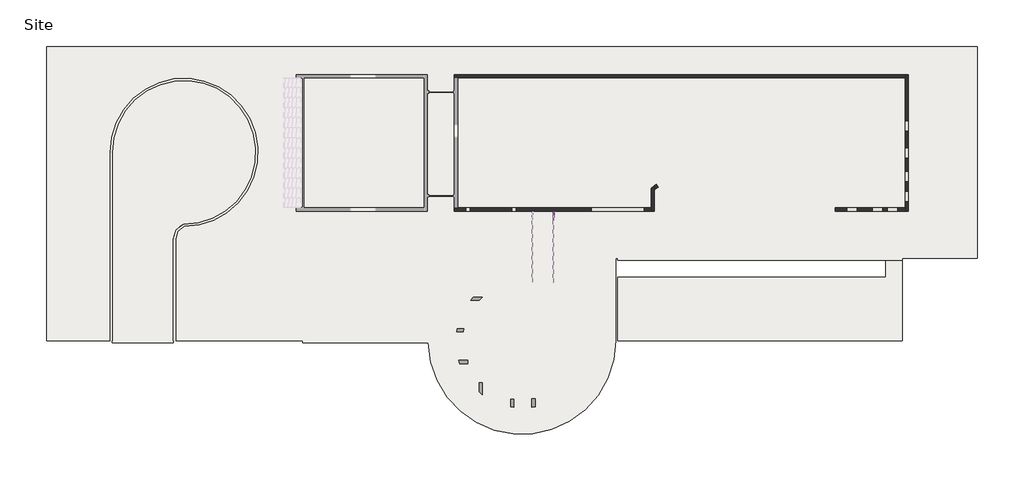
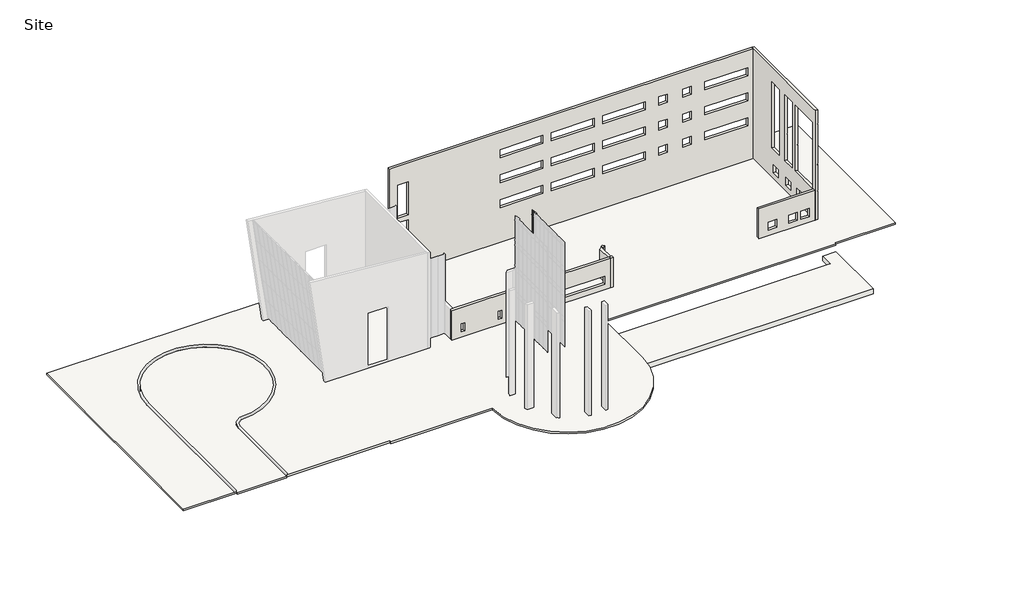
# One storey, part 4 of 4: 17 members, 6 walls, 3 plates, 3 slabs.
"""IFC4 building model written with IfcOpenShell, lengths in millimetres."""

import ifcopenshell
import ifcopenshell.guid

model = None  # the IFC model being written
_history = None  # IfcOwnerHistory: only IFC2X3 demands one
_inside = {}  # id of a spatial element -> (the spatial element, [elements in it])
_under = {}  # id of a project, library or spatial element -> (it, [spatial elements below it])
_declared = {}  # id of a project -> (the project, [libraries it declares])
_typed = {}  # id of a type object -> (the type object, [elements of that type])
_made_of = {}  # id of a material, layer set ... -> (it, [elements and type objects made of it])


def new_model(schema):
    """Start an empty IFC model of exactly this schema.

    Asked for "IFC4X3", IfcOpenShell would pick the latest addendum, in which some entities
    have other attributes; the version numbers below select the first issue.
    IFC2X3 requires an IfcOwnerHistory on every rooted entity: one is made here for all.
    """
    global model, _history
    if schema == "IFC4X3":
        model = ifcopenshell.file(schema_version=(4, 3, 0, 0))
    else:
        model = ifcopenshell.file(schema=schema)
    _inside.clear()
    _under.clear()
    _declared.clear()
    _typed.clear()
    _made_of.clear()
    _history = None
    if model.schema == "IFC2X3":
        org = make("IfcOrganization", Name="unknown")
        user = make(
            "IfcPersonAndOrganization",
            ThePerson=make("IfcPerson", FamilyName="unknown"),
            TheOrganization=org,
        )
        app = make(
            "IfcApplication",
            ApplicationDeveloper=org,
            Version="unknown",
            ApplicationFullName="unknown",
            ApplicationIdentifier="unknown",
        )
        _history = make(
            "IfcOwnerHistory",
            OwningUser=user,
            OwningApplication=app,
            ChangeAction="ADDED",
            CreationDate=0,
        )
    return model


def make(cls, **values):
    """One entity of the class cls with the attributes given. An attribute that is None is left unset."""
    return model.create_entity(
        cls, **{name: value for name, value in values.items() if value is not None}
    )


def rooted(cls, **values):
    """An entity with a GlobalId (a new one), such as an element, a storey or a relation."""
    return make(cls, GlobalId=ifcopenshell.guid.new(), OwnerHistory=_history, **values)


def si_unit(unit_type, name, prefix=None):
    """IfcSIUnit, for example si_unit("LENGTHUNIT", "METRE", prefix="MILLI")."""
    return make("IfcSIUnit", UnitType=unit_type, Prefix=prefix, Name=name)


def assignment(units):
    """IfcUnitAssignment: the units of a project."""
    return None if units is None else make("IfcUnitAssignment", Units=units)


def point(xyz):
    """IfcCartesianPoint."""
    return None if xyz is None else make("IfcCartesianPoint", Coordinates=xyz)


def direction(xyz):
    """IfcDirection."""
    return None if xyz is None else make("IfcDirection", DirectionRatios=xyz)


def frame(location, z_axis=None, x_axis=None):
    """IfcAxis2Placement3D, a coordinate frame: its origin and axes. An axis left out is left unset."""
    return make(
        "IfcAxis2Placement3D",
        Location=point(location),
        Axis=direction(z_axis),
        RefDirection=direction(x_axis),
    )


def frame_2d(location, x_axis=None):
    """IfcAxis2Placement2D, a coordinate frame in the plane: its origin and x axis."""
    return make(
        "IfcAxis2Placement2D", Location=point(location), RefDirection=direction(x_axis)
    )


def origin():
    """The frame at (0, 0, 0) with its axes left unset."""
    return frame((0.0, 0.0, 0.0))


def origin_with_axes():
    """The frame at (0, 0, 0) with the z axis (0, 0, 1) and the x axis (1, 0, 0) written out."""
    return frame((0.0, 0.0, 0.0), z_axis=(0.0, 0.0, 1.0), x_axis=(1.0, 0.0, 0.0))


def place(relative_to, where):
    """IfcLocalPlacement: puts the frame where relative to a parent placement (None: the world)."""
    return make(
        "IfcLocalPlacement", PlacementRelTo=relative_to, RelativePlacement=where
    )


def context(
    kind, dimensions, precision=None, world=None, true_north=None, identifier=None
):
    """IfcGeometricRepresentationContext, for example the 3D "Model" context."""
    return make(
        "IfcGeometricRepresentationContext",
        ContextIdentifier=identifier,
        ContextType=kind,
        CoordinateSpaceDimension=dimensions,
        Precision=precision,
        WorldCoordinateSystem=world,
        TrueNorth=true_north,
    )


def project(units=None, contexts=None):
    """IfcProject with its units and contexts."""
    return rooted(
        "IfcProject",
        Name="project",
        RepresentationContexts=contexts,
        UnitsInContext=assignment(units),
    )


def spatial(cls, under=None, at=None, **own):
    """A site, building, storey or space (cls), placed at a placement, below another one or the project."""
    s = rooted(cls, ObjectPlacement=at, **own)
    if under is not None:
        _under.setdefault(under.id(), (under, []))[1].append(s)
    return s


def polyline(points):
    """IfcPolyline through the points."""
    return make("IfcPolyline", Points=[point(p) for p in points])


def circle_curve(where, radius):
    """IfcCircle in the frame where."""
    return make("IfcCircle", Position=where, Radius=radius)


def trimmed(basis, trim1, trim2, sense, master):
    """IfcTrimmedCurve: the piece of a basis curve between two trims."""
    return make(
        "IfcTrimmedCurve",
        BasisCurve=basis,
        Trim1=trim1,
        Trim2=trim2,
        SenseAgreement=sense,
        MasterRepresentation=master,
    )


def segment(curve, same_sense, transition):
    """IfcCompositeCurveSegment."""
    return make(
        "IfcCompositeCurveSegment",
        Transition=transition,
        SameSense=same_sense,
        ParentCurve=curve,
    )


def composite_curve(segments, self_intersect=None):
    """IfcCompositeCurve: segments joined end to end."""
    return make("IfcCompositeCurve", Segments=segments, SelfIntersect=self_intersect)


def outline(outer, holes=None, kind="AREA"):
    """IfcArbitraryClosedProfileDef: a profile drawn as a closed curve; with holes, ...WithVoids."""
    if holes is None:
        return make("IfcArbitraryClosedProfileDef", ProfileType=kind, OuterCurve=outer)
    return make(
        "IfcArbitraryProfileDefWithVoids",
        ProfileType=kind,
        OuterCurve=outer,
        InnerCurves=holes,
    )


def extrude(swept, where, along, depth):
    """IfcExtrudedAreaSolid: the profile swept, set in the frame where, extruded along a direction by depth."""
    return make(
        "IfcExtrudedAreaSolid",
        SweptArea=swept,
        Position=where,
        ExtrudedDirection=direction(along),
        Depth=depth,
    )


def faces_of(points, faces, orient=None, outer=None):
    """IfcFace entities. A face is a list of loops; a loop is a list of indices into points, from 0.

    orient and outer hold one flag for each loop. By default every Orientation is true, the
    first loop of a face is its IfcFaceOuterBound and the others are IfcFaceBound.
    """
    made = []
    for i, loops in enumerate(faces):
        bounds = []
        for j, loop in enumerate(loops):
            is_outer = j == 0 if outer is None else outer[i][j]
            bounds.append(
                make(
                    "IfcFaceOuterBound" if is_outer else "IfcFaceBound",
                    Bound=make("IfcPolyLoop", Polygon=[points[k] for k in loop]),
                    Orientation=True if orient is None else orient[i][j],
                )
            )
        made.append(make("IfcFace", Bounds=bounds))
    return made


def faceted_brep(points, faces, orient=None, outer=None, voids=None):
    """IfcFacetedBrep: a solid bounded by flat faces; with voids (closed shells), ...WithVoids."""
    shared = [point(p) for p in points]
    hull = make("IfcClosedShell", CfsFaces=faces_of(shared, faces, orient, outer))
    if voids is None:
        return make("IfcFacetedBrep", Outer=hull)
    return make(
        "IfcFacetedBrepWithVoids",
        Outer=hull,
        Voids=[
            make(cls, CfsFaces=faces_of(shared, fs, o, b)) for cls, fs, o, b in voids
        ],
    )


def shape(context_of_items, identifier, shape_type, items):
    """IfcShapeRepresentation: the items that make up one representation, for example the "Body"."""
    return make(
        "IfcShapeRepresentation",
        ContextOfItems=context_of_items,
        RepresentationIdentifier=identifier,
        RepresentationType=shape_type,
        Items=items,
    )


def source(mapping_origin, context_of_items, identifier, shape_type, items):
    """IfcRepresentationMap: a shape defined once, which mapped items show again and again."""
    return make(
        "IfcRepresentationMap",
        MappingOrigin=mapping_origin,
        MappedRepresentation=shape(context_of_items, identifier, shape_type, items),
    )


def transform(
    local_origin,
    x_axis=None,
    y_axis=None,
    z_axis=None,
    scale=None,
    scale2=None,
    scale3=None,
    uniform=True,
):
    """IfcCartesianTransformationOperator3D, or its non-uniform kind. x_axis, y_axis, z_axis: its Axis1, 2, 3."""
    if uniform:
        return make(
            "IfcCartesianTransformationOperator3D",
            Axis1=direction(x_axis),
            Axis2=direction(y_axis),
            LocalOrigin=point(local_origin),
            Scale=scale,
            Axis3=direction(z_axis),
        )
    return make(
        "IfcCartesianTransformationOperator3DnonUniform",
        Axis1=direction(x_axis),
        Axis2=direction(y_axis),
        LocalOrigin=point(local_origin),
        Scale=scale,
        Axis3=direction(z_axis),
        Scale2=scale2,
        Scale3=scale3,
    )


def mapped(mapping_source, mapping_target):
    """IfcMappedItem: shows the shape of a source again, moved by a transform."""
    return make(
        "IfcMappedItem", MappingSource=mapping_source, MappingTarget=mapping_target
    )


def made_of(thing, what):
    """Note that an element or type object is made of a material, layer set ...; save() writes the relation."""
    if what is not None:
        _made_of.setdefault(what.id(), (what, []))[1].append(thing)
    return thing


def element(
    cls,
    number,
    at=None,
    inside=None,
    cuts=None,
    type_object=None,
    material=None,
    context=None,
    identifier="Body",
    shape_type=None,
    held_by="IfcProductDefinitionShape",
    body=None,
    shapes=None,
    **own,
):
    """One element of the class cls, such as IfcWall. Its Tag is "e" and its number.

    at: its placement. inside: the storey or other place that contains it. cuts: it is an
    opening in that element (IfcRelVoidsElement). A single representation is given by context,
    identifier, shape_type and body (its items); several are given by shapes. held_by: the class
    of the entity that holds the representations. save() writes the other relations.
    """
    e = rooted(cls, Tag="e%d" % number, ObjectPlacement=at, **own)
    if body is not None:
        shapes = [shape(context, identifier, shape_type, body)]
    if shapes is not None:
        e.Representation = make(held_by, Representations=shapes)
    if inside is not None:
        _inside.setdefault(inside.id(), (inside, []))[1].append(e)
    if cuts is not None:
        rooted(
            "IfcRelVoidsElement", RelatingBuildingElement=cuts, RelatedOpeningElement=e
        )
    if type_object is not None:
        _typed.setdefault(type_object.id(), (type_object, []))[1].append(e)
    return made_of(e, material)


def aggregate(whole, parts):
    """IfcRelAggregates: a whole, such as a stair, and the parts it consists of."""
    return rooted("IfcRelAggregates", RelatingObject=whole, RelatedObjects=parts)


def save(model, path):
    """Write the relations noted so far, then the file.

    IfcRelAggregates (storeys below a building ...), IfcRelContainedInSpatialStructure (elements
    in a storey), IfcRelDefinesByType, IfcRelAssociatesMaterial and IfcRelDeclares: one each for
    every whole, place, type object, material and project.
    """
    for whole, parts in _under.values():
        aggregate(whole, parts)
    for where, things in _inside.values():
        rooted(
            "IfcRelContainedInSpatialStructure",
            RelatedElements=things,
            RelatingStructure=where,
        )
    for kind, things in _typed.values():
        rooted("IfcRelDefinesByType", RelatedObjects=things, RelatingType=kind)
    for what, things in _made_of.values():
        rooted("IfcRelAssociatesMaterial", RelatedObjects=things, RelatingMaterial=what)
    for by, libraries in _declared.values():
        rooted("IfcRelDeclares", RelatingContext=by, RelatedDefinitions=libraries)
    model.write(path)


def plane_surface(at):
    """IfcPlane: the flat surface through the origin of the frame at, square to its z axis."""
    return make("IfcPlane", Position=at)


def cylinder_surface(at, radius):
    """IfcCylindricalSurface: all points at the distance radius from the z axis of the frame at."""
    return make("IfcCylindricalSurface", Position=at, Radius=radius)


def revolved_surface(curve, axis_point, axis_direction):
    """IfcSurfaceOfRevolution: the curve turned about the line through axis_point along axis_direction."""
    return make(
        "IfcSurfaceOfRevolution",
        SweptCurve=make("IfcArbitraryOpenProfileDef", ProfileType="CURVE", Curve=curve),
        AxisPosition=make("IfcAxis1Placement", Location=point(axis_point), Axis=direction(axis_direction)),
    )


def advanced_brep(points, edges, surfaces, faces):
    """IfcAdvancedBrep: a solid bounded by faces that lie on surfaces and meet in shared edges.

    An edge is (start, end): straight between two places in points (the first is 0);
    or (start, end, curve); or (start, end, curve, False) where it runs against its curve.
    A face is (place in surfaces, loops), or (place, loops, False) where it looks against
    its surface's normal. A loop lists edges by number (the first is 1), with a minus sign
    where the edge is run from its end to its start. The first loop is the outer one.
    """
    corners = [point(p) for p in points]
    vertices = [make("IfcVertexPoint", VertexGeometry=c) for c in corners]
    made = []
    for start, end, *more in edges:
        made.append(
            make(
                "IfcEdgeCurve",
                EdgeStart=vertices[start],
                EdgeEnd=vertices[end],
                EdgeGeometry=more[0] if more else make("IfcPolyline", Points=[corners[start], corners[end]]),
                SameSense=more[1] if len(more) > 1 else True,
            )
        )
    hull = []
    for where, loops, *sense in faces:
        bounds = []
        for j, loop in enumerate(loops):
            ring = [make("IfcOrientedEdge", EdgeElement=made[abs(k) - 1], Orientation=k > 0) for k in loop]
            bounds.append(
                make(
                    "IfcFaceOuterBound" if j == 0 else "IfcFaceBound",
                    Bound=make("IfcEdgeLoop", EdgeList=ring),
                    Orientation=True,
                )
            )
        hull.append(make("IfcAdvancedFace", Bounds=bounds, FaceSurface=surfaces[where], SameSense=sense[0] if sense else True))
    return make("IfcAdvancedBrep", Outer=make("IfcClosedShell", CfsFaces=hull))


def member_5d07894b(model_context):
    return source(origin(), model_context, "Body", "SweptSolid", [
        extrude(outline(polyline([(31.75, 63.5), (31.75, -63.5), (-31.75, -63.5), (-31.75, 63.5), (31.75, 63.5)])), frame((0.0, 0.0, -4629.15), z_axis=(0.0, 0.0, 1.0), x_axis=(1.0, 0.0, 0.0)), (0.0, 0.0, 1.0), 4629.15),
    ])


def member_3ba9e939(model_context):
    return source(origin(), model_context, "Body", "SweptSolid", [
        extrude(outline(polyline([(31.75, 63.5), (31.75, -63.5), (-31.75, -63.5), (-31.75, 63.5), (31.75, 63.5)])), frame((0.0, 0.0, -3746.5), z_axis=(0.0, 0.0, 1.0), x_axis=(1.0, 0.0, 0.0)), (0.0, 0.0, 1.0), 3746.5),
    ])


def member_ad567e07(model_context):
    return source(origin(), model_context, "Body", "SweptSolid", [
        extrude(outline(polyline([(31.75, 63.5), (31.75, -63.5), (-31.75, -63.5), (-31.75, 63.5), (31.75, 63.5)])), frame((0.0, 0.0, -819.15), z_axis=(0.0, 0.0, 1.0), x_axis=(1.0, 0.0, 0.0)), (0.0, 0.0, 1.0), 819.15),
    ])


def member_7db1855a(model_context):
    return source(origin(), model_context, "Body", "SweptSolid", [
        extrude(outline(polyline([(31.75, 63.5), (31.75, -63.5), (-31.75, -63.5), (-31.75, 63.5), (31.75, 63.5)])), frame((0.0, 0.0, -850.9), z_axis=(0.0, 0.0, 1.0), x_axis=(1.0, 0.0, 0.0)), (0.0, 0.0, 1.0), 850.9),
    ])


def member_ffd4c858(model_context):
    return source(origin(), model_context, "Body", "SweptSolid", [
        extrude(outline(polyline([(31.75, 63.5), (31.75, -63.5), (-31.75, -63.5), (-31.75, 63.5), (31.75, 63.5)])), frame((0.0, 0.0, -457.2), z_axis=(0.0, 0.0, 1.0), x_axis=(1.0, 0.0, 0.0)), (0.0, 0.0, 1.0), 457.2),
    ])


def member_15823cb3(model_context):
    return source(origin(), model_context, "Body", "SweptSolid", [
        extrude(outline(polyline([(0.0, 63.5), (0.0, -63.5), (-63.5, -63.5), (-63.5, 63.5), (0.0, 63.5)])), frame((0.0, 0.0, -457.2), z_axis=(0.0, 0.0, 1.0), x_axis=(1.0, 0.0, 0.0)), (0.0, 0.0, 1.0), 457.2),
    ])


def member_e9605c56(model_context):
    return source(origin(), model_context, "Body", "SweptSolid", [
        extrude(outline(polyline([(0.0, 63.5), (0.0, -63.5), (-63.5, -63.5), (-63.5, 63.5), (0.0, 63.5)])), frame((0.0, 0.0, -825.5), z_axis=(0.0, 0.0, 1.0), x_axis=(1.0, 0.0, 0.0)), (0.0, 0.0, 1.0), 825.5),
    ])


def system_panel_glazed_5cc7900c(model_context):
    return source(origin(), model_context, "Body", "SweptSolid", [
        extrude(outline(polyline([(180.975, 19.05), (-180.975, 19.05), (-180.975, 44.45), (180.975, 44.45), (180.975, 19.05)])), origin_with_axes(), (0.0, 0.0, 1.0), 850.9),
    ])


def system_panel_glazed_032e4dab(model_context):
    return source(origin(), model_context, "Body", "SweptSolid", [
        extrude(outline(polyline([(180.975, 19.05), (-180.975, 19.05), (-180.975, 44.45), (180.975, 44.45), (180.975, 19.05)])), origin_with_axes(), (0.0, 0.0, 1.0), 3746.5),
    ])


def system_panel_glazed_cc98a0ec(model_context):
    return source(origin(), model_context, "Body", "SweptSolid", [
        extrude(outline(polyline([(180.975, 19.05), (-180.975, 19.05), (-180.975, 44.45), (180.975, 44.45), (180.975, 19.05)])), origin_with_axes(), (0.0, 0.0, 1.0), 819.15),
    ])


model = new_model("IFC4")

# Units and contexts
model_context = context("Model", 3, world=origin())
ifc_project = project(units=[si_unit("LENGTHUNIT", "METRE", prefix="MILLI")], contexts=[model_context])

# Site, building, storey
site = spatial("IfcSite", under=ifc_project)
building = spatial("IfcBuilding", under=site)
storey = spatial("IfcBuildingStorey", under=building, Name="Site", Elevation=-152.4)

# Members
placement = place(None, origin())
member_shape = member_5d07894b(model_context)
element("IfcMember", 1, ObjectType="Rectangular Mullion1 : 2.5\" x 5\" rectangular", at=placement, inside=storey, context=model_context, shape_type="MappedRepresentation", body=[
    mapped(member_shape, transform((10878.8276119, 37629.311889, -88.9), x_axis=(0.0, 1.0, 0.0), y_axis=(1.0, 0.0, 0.0), z_axis=(0.0, 0.0, -1.0))),
])
member_2_shape = member_3ba9e939(model_context)
element("IfcMember", 2, ObjectType="Rectangular Mullion1 : 2.5\" x 5\" rectangular", at=placement, inside=storey, context=model_context, shape_type="MappedRepresentation", body=[
    mapped(member_2_shape, transform((10878.8276119, 37629.311889, 5518.15), x_axis=(0.0, 1.0, 0.0), y_axis=(1.0, 0.0, 0.0), z_axis=(0.0, 0.0, -1.0))),
])
element("IfcMember", 3, ObjectType="Rectangular Mullion1 : 2.5\" x 5\" rectangular", at=placement, inside=storey, context=model_context, shape_type="MappedRepresentation", body=[
    mapped(member_2_shape, transform((10878.8276119, 37629.311889, 10242.55), x_axis=(0.0, 1.0, 0.0), y_axis=(1.0, 0.0, 0.0), z_axis=(0.0, 0.0, -1.0))),
])
element("IfcMember", 4, ObjectType="Rectangular Mullion1 : 2.5\" x 5\" rectangular", at=placement, inside=storey, context=model_context, shape_type="MappedRepresentation", body=[
    mapped(member_2_shape, transform((10878.8276119, 37629.311889, 14966.95), x_axis=(0.0, 1.0, 0.0), y_axis=(1.0, 0.0, 0.0), z_axis=(0.0, 0.0, -1.0))),
])
member_3_shape = member_ad567e07(model_context)
element("IfcMember", 5, ObjectType="Rectangular Mullion1 : 2.5\" x 5\" rectangular", at=placement, inside=storey, context=model_context, shape_type="MappedRepresentation", body=[
    mapped(member_3_shape, transform((10878.8276119, 37629.311889, 18776.95), x_axis=(0.0, 1.0, 0.0), y_axis=(1.0, 0.0, 0.0), z_axis=(0.0, 0.0, -1.0))),
])
member_4_shape = member_7db1855a(model_context)
element("IfcMember", 6, ObjectType="Rectangular Mullion1 : 2.5\" x 5\" rectangular", at=placement, inside=storey, context=model_context, shape_type="MappedRepresentation", body=[
    mapped(member_4_shape, transform((10878.8276119, 37629.311889, 14052.55), x_axis=(0.0, 1.0, 0.0), y_axis=(1.0, 0.0, 0.0), z_axis=(0.0, 0.0, -1.0))),
])
element("IfcMember", 7, ObjectType="Rectangular Mullion1 : 2.5\" x 5\" rectangular", at=placement, inside=storey, context=model_context, shape_type="MappedRepresentation", body=[
    mapped(member_4_shape, transform((10878.8276119, 37629.311889, 4603.75), x_axis=(0.0, 1.0, 0.0), y_axis=(1.0, 0.0, 0.0), z_axis=(0.0, 0.0, -1.0))),
])
element("IfcMember", 8, ObjectType="Rectangular Mullion1 : 2.5\" x 5\" rectangular", at=placement, inside=storey, context=model_context, shape_type="MappedRepresentation", body=[
    mapped(member_4_shape, transform((10878.8276119, 37629.311889, 9328.15), x_axis=(0.0, 1.0, 0.0), y_axis=(1.0, 0.0, 0.0), z_axis=(0.0, 0.0, -1.0))),
])
member_5_shape = member_ffd4c858(model_context)
element("IfcMember", 9, ObjectType="Rectangular Mullion1 : 2.5\" x 5\" rectangular", at=placement, inside=storey, context=model_context, shape_type="MappedRepresentation", body=[
    mapped(member_5_shape, transform((10878.8276119, 38086.511889, 14935.2), x_axis=(0.0, 0.0, 1.0), y_axis=(1.0, 0.0, 0.0), z_axis=(0.0, 1.0, 0.0))),
])
element("IfcMember", 10, ObjectType="Rectangular Mullion1 : 2.5\" x 5\" rectangular", at=placement, inside=storey, context=model_context, shape_type="MappedRepresentation", body=[
    mapped(member_5_shape, transform((10878.8276119, 38086.511889, 10210.8), x_axis=(0.0, 0.0, 1.0), y_axis=(1.0, 0.0, 0.0), z_axis=(0.0, 1.0, 0.0))),
])
element("IfcMember", 11, ObjectType="Rectangular Mullion1 : 2.5\" x 5\" rectangular", at=placement, inside=storey, context=model_context, shape_type="MappedRepresentation", body=[
    mapped(member_5_shape, transform((10878.8276119, 38086.511889, 5486.4), x_axis=(0.0, 0.0, 1.0), y_axis=(1.0, 0.0, 0.0), z_axis=(0.0, 1.0, 0.0))),
])
element("IfcMember", 12, ObjectType="Rectangular Mullion1 : 2.5\" x 5\" rectangular", at=placement, inside=storey, context=model_context, shape_type="MappedRepresentation", body=[
    mapped(member_5_shape, transform((10878.8276119, 38086.511889, 9296.4), x_axis=(0.0, 0.0, 1.0), y_axis=(1.0, 0.0, 0.0), z_axis=(0.0, 1.0, 0.0))),
])
element("IfcMember", 13, ObjectType="Rectangular Mullion1 : 2.5\" x 5\" rectangular", at=placement, inside=storey, context=model_context, shape_type="MappedRepresentation", body=[
    mapped(member_5_shape, transform((10878.8276119, 38086.511889, 4572.0), x_axis=(0.0, 0.0, 1.0), y_axis=(1.0, 0.0, 0.0), z_axis=(0.0, 1.0, 0.0))),
])
element("IfcMember", 14, ObjectType="Rectangular Mullion1 : 2.5\" x 5\" rectangular", at=placement, inside=storey, context=model_context, shape_type="MappedRepresentation", body=[
    mapped(member_5_shape, transform((10878.8276119, 38086.511889, 14020.8), x_axis=(0.0, 0.0, 1.0), y_axis=(1.0, 0.0, 0.0), z_axis=(0.0, 1.0, 0.0))),
])
element("IfcMember", 15, ObjectType="Rectangular Mullion1 : 2.5\" x 5\" rectangular", at=placement, inside=storey, context=model_context, shape_type="MappedRepresentation", body=[
    mapped(member_5_shape, transform((10878.8276119, 38086.511889, 18745.2), x_axis=(0.0, 0.0, 1.0), y_axis=(1.0, 0.0, 0.0), z_axis=(0.0, 1.0, 0.0))),
])
member_6_shape = member_15823cb3(model_context)
element("IfcMember", 16, ObjectType="Rectangular Mullion1 : 2.5\" x 5\" rectangular", at=placement, inside=storey, context=model_context, shape_type="MappedRepresentation", body=[
    mapped(member_6_shape, transform((10878.8276119, 37629.311889, -152.4), x_axis=(0.0, 0.0, -1.0), y_axis=(1.0, 0.0, 0.0), z_axis=(0.0, -1.0, 0.0))),
])
member_7_shape = member_e9605c56(model_context)
element("IfcMember", 17, ObjectType="Rectangular Mullion1 : 2.5\" x 5\" rectangular", at=placement, inside=storey, context=model_context, shape_type="MappedRepresentation", body=[
    mapped(member_7_shape, transform((10878.8276119, 37629.311889, 19659.6), x_axis=(0.0, 0.0, 1.0), y_axis=(1.0, 0.0, 0.0), z_axis=(0.0, 1.0, 0.0))),
])

# Plates
system_panel_glazed_shape = system_panel_glazed_5cc7900c(model_context)
element("IfcPlate", 18, ObjectType="System Panel : Glazed", at=placement, inside=storey, context=model_context, shape_type="MappedRepresentation", body=[
    mapped(system_panel_glazed_shape, transform((10878.8276119, 37842.036889, 14052.55), x_axis=(0.0, 1.0, 0.0), y_axis=(-1.0, 0.0, 0.0), z_axis=(0.0, 0.0, 1.0))),
])
system_panel_glazed_2_shape = system_panel_glazed_032e4dab(model_context)
element("IfcPlate", 19, ObjectType="System Panel : Glazed", at=placement, inside=storey, context=model_context, shape_type="MappedRepresentation", body=[
    mapped(system_panel_glazed_2_shape, transform((10878.8276119, 37842.036889, 14966.95), x_axis=(0.0, 1.0, 0.0), y_axis=(-1.0, 0.0, 0.0), z_axis=(0.0, 0.0, 1.0))),
])
system_panel_glazed_3_shape = system_panel_glazed_cc98a0ec(model_context)
element("IfcPlate", 20, ObjectType="System Panel : Glazed", at=placement, inside=storey, context=model_context, shape_type="MappedRepresentation", body=[
    mapped(system_panel_glazed_3_shape, transform((10878.8276119, 37842.036889, 18776.95), x_axis=(0.0, 1.0, 0.0), y_axis=(-1.0, 0.0, 0.0), z_axis=(0.0, 0.0, 1.0))),
])

# Slabs
element("IfcSlab", 21, ObjectType="a_drive", at=placement, inside=storey, context=model_context, shape_type="SweptSolid", body=[
    extrude(outline(composite_curve([segment(trimmed(circle_curve(frame_2d((-42359.2307976, 46620.911889)), 10363.2), [point((-52722.4307976, 46620.911889))], [point((-42384.6461103, 36257.743054))], False, "CARTESIAN"), True, "CONTINUOUS"), segment(trimmed(circle_curve(frame_2d((-41679.1721267, 34169.1174245)), 2204.5522361), [point((-42384.6461103, 36257.743054))], [point((-43883.2307976, 34122.4704857))], True, "CARTESIAN"), True, "CONTINUOUS"), segment(polyline([(-43883.2307976, 34122.4704857), (-43883.2307976, 19188.911889), (-52722.4307976, 19188.911889), (-52722.4307976, 46620.911889)]), True, "CONTINUOUS")], self_intersect=False)), frame((0.0, 0.0, -457.2), z_axis=(0.0, 0.0, 1.0), x_axis=(1.0, 0.0, 0.0)), (0.0, 0.0, 1.0), 304.8),
])
element("IfcSlab", 22, ObjectType="a_site paving", at=placement, inside=storey, context=model_context, shape_type="SweptSolid", body=[
    extrude(outline(composite_curve([segment(polyline([(71940.7692024, 61860.911889), (71940.7692024, 31380.911889), (61120.3692024, 31380.911889), (61120.3692024, 31076.111889), (20124.7692024, 31076.111889), (20124.7692024, 31380.911889), (19819.9692024, 31380.911889), (19819.9692024, 19493.711889)]), True, "CONTINUOUS"), segment(trimmed(circle_curve(frame_2d((6332.9997246, 19493.711889)), 13486.9694778), [point((19819.9692024, 19493.711889))], [point((-7150.5251356, 19188.911889))], False, "CARTESIAN"), True, "CONTINUOUS"), segment(polyline([(-7150.5251356, 19188.911889), (-25290.4307976, 19188.911889), (-25290.4307976, 19493.711889), (-43883.2307976, 19493.711889), (-43883.2307976, 34122.4704857)]), True, "CONTINUOUS"), segment(trimmed(circle_curve(frame_2d((-41679.1721267, 34169.1174245)), 2204.5522361), [point((-43883.2307976, 34122.4704857))], [point((-42384.6461103, 36257.743054))], False, "CARTESIAN"), True, "CONTINUOUS"), segment(trimmed(circle_curve(frame_2d((-42359.2307976, 46620.911889)), 10363.2), [point((-42384.6461103, 36257.743054))], [point((-52722.4307976, 46620.911889))], True, "CARTESIAN"), True, "CONTINUOUS"), segment(polyline([(-52722.4307976, 46620.911889), (-52722.4307976, 19493.711889), (-62171.2307976, 19493.711889), (-62171.2307976, 61860.911889), (71940.7692024, 61860.911889)]), True, "CONTINUOUS")], self_intersect=False)), frame((0.0, 0.0, -457.2), z_axis=(0.0, 0.0, 1.0), x_axis=(1.0, 0.0, 0.0)), (0.0, 0.0, 1.0), 304.8),
])
element("IfcSlab", 23, ObjectType="water feature", at=placement, inside=storey, context=model_context, shape_type="SweptSolid", body=[
    extrude(outline(polyline([(20124.7692024, 28656.761889), (58732.7692024, 28656.761889), (58732.7692024, 31076.111889), (61120.3692024, 31076.111889), (61120.3692024, 19493.711889), (20124.7692024, 19493.711889), (20124.7692024, 28656.761889)])), frame((0.0, 0.0, -2590.8), z_axis=(0.0, 0.0, 1.0), x_axis=(1.0, 0.0, 0.0)), (0.0, 0.0, 1.0), 914.4),
])

# Walls
element("IfcWall", 24, ObjectType="Stone on CMU", at=placement, inside=storey, context=model_context, shape_type="AdvancedBrep", body=[
    advanced_brep(
    [(24926.9567024, 41466.5312272, -152.4), (24926.9567024, 38618.324389, -152.4), (24926.9567024, 38164.299389, -152.4), (24926.9567024, 38164.299389, 5486.4), (24926.9567024, 38618.324389, 5486.4), (24926.9567024, 38618.324389, 5181.6), (24926.9567024, 41466.5312272, 5181.6), (25380.9817024, 41789.4772012, -152.4), (25380.9817024, 41789.4772012, 5181.6), (25380.9817024, 38618.324389, 5181.6), (25380.9817024, 38618.324389, 5486.4), (25380.9817024, 38164.299389, 5486.4), (25380.9817024, 38164.299389, -152.4), (25380.9817024, 41234.3316602, -152.4)],
    [
        (0, 1),
        (1, 2),
        (2, 3),
        (3, 4),
        (4, 5),
        (5, 6),
        (6, 0),
        (7, 8),
        (8, 9),
        (9, 10),
        (10, 11),
        (11, 12),
        (12, 13),
        (13, 7),
        (0, 7, circle_curve(frame((38486.136956, 22884.5054507, -152.4), z_axis=(0.0, 0.0, -1.0), x_axis=(1.0, 0.0, 0.0)), 23003.1095965)),
        (12, 2),
        (3, 11),
        (10, 4),
        (9, 5),
        (8, 6, circle_curve(frame((38486.136956, 22884.5054507, 5181.6), z_axis=(0.0, 0.0, 1.0), x_axis=(1.0, 0.0, 0.0)), 23003.1095965)),
    ],
    [
        plane_surface(frame((24926.9567024, 41350.796414, -152.4), z_axis=(-1.0, 0.0, 0.0), x_axis=(0.0, -1.0, 0.0))),
        plane_surface(frame((25380.9817024, 41350.796414, -152.4), z_axis=(1.0, 0.0, 0.0), x_axis=(0.0, 1.0, 0.0))),
        plane_surface(frame((24926.9567024, 41350.796414, -152.4), z_axis=(0.0, 0.0, -1.0), x_axis=(1.0, 0.0, 0.0))),
        plane_surface(frame((24926.9567024, 38391.311889, 5486.4), z_axis=(0.0, 0.0, 1.0), x_axis=(1.0, 0.0, 0.0))),
        plane_surface(frame((24926.9567024, 38618.324389, 5486.4), z_axis=(0.0, 1.0, 0.0), x_axis=(1.0, 0.0, 0.0))),
        plane_surface(frame((24926.9567024, 38618.324389, 5181.6), z_axis=(0.0, 0.0, 1.0), x_axis=(1.0, 0.0, 0.0))),
        plane_surface(frame((24696.7692024, 38164.299389, -152.4), z_axis=(0.0, -1.0, 0.0), x_axis=(1.0, 0.0, 0.0))),
        cylinder_surface(frame((38486.136956, 22884.5054507, -152.4), z_axis=(0.0, 0.0, 1.0), x_axis=(1.0, 0.0, 0.0)), 23003.1095965),
    ],
    [
        (0, [[1, 2, 3, 4, 5, 6, 7]]),
        (1, [[8, 9, 10, 11, 12, 13, 14]]),
        (2, [[-2, -1, 15, -14, -13, 16]]),
        (3, [[-4, 17, -11, 18]]),
        (4, [[-5, -18, -10, 19]]),
        (5, [[-6, -19, -9, 20]]),
        (6, [[-3, -16, -12, -17]]),
        (7, [[-7, -20, -8, -15]]),
    ],
),
])
element("IfcWall", 25, ObjectType="Stone on CMU", at=placement, inside=storey, context=model_context, shape_type="Brep", body=[
    faceted_brep([(24926.9567024, 38618.324389, 5486.4), (6799.2942024, 38618.324389, 5486.4), (6656.4192024, 38618.324389, 5486.4), (-2965.7977165, 38618.324389, 5486.4), (-3419.8227165, 38618.324389, 5486.4), (-3419.8227165, 38164.299389, 5486.4), (24926.9567024, 38164.299389, 5486.4), (24926.9567024, 38618.324389, -152.4), (-2965.7977165, 38618.324389, -152.4), (-3419.8227165, 38618.324389, -152.4), (24926.9567024, 38618.324389, 5181.6), (4884.7692024, 38618.324389, 2438.4), (4884.7692024, 38618.324389, 914.4), (5494.3692024, 38618.324389, 914.4), (5494.3692024, 38618.324389, 2438.4), (-1750.9807976, 38618.324389, 2438.4), (-1750.9807976, 38618.324389, 914.4), (-1141.3807976, 38618.324389, 914.4), (-1141.3807976, 38618.324389, 2438.4), (16314.7692024, 38618.324389, 914.4), (23934.7692024, 38618.324389, 914.4), (23934.7692024, 38618.324389, 2438.4), (16314.7692024, 38618.324389, 2438.4), (24926.9567024, 38164.299389, -152.4), (-3419.8227165, 38164.299389, -152.4), (4884.7692024, 38164.299389, 2438.4), (5494.3692024, 38164.299389, 2438.4), (5494.3692024, 38164.299389, 914.4), (4884.7692024, 38164.299389, 914.4), (-1750.9807976, 38164.299389, 2438.4), (-1141.3807976, 38164.299389, 2438.4), (-1141.3807976, 38164.299389, 914.4), (-1750.9807976, 38164.299389, 914.4), (16314.7692024, 38164.299389, 914.4), (16314.7692024, 38164.299389, 2438.4), (23934.7692024, 38164.299389, 2438.4), (23934.7692024, 38164.299389, 914.4)], [[[0, 1, 2, 3, 4, 5, 6]], [[7, 8, 9, 4, 3, 2, 1, 0, 10], [11, 12, 13, 14], [15, 16, 17, 18], [19, 20, 21, 22]], [[23, 6, 5, 24], [25, 26, 27, 28], [29, 30, 31, 32], [33, 34, 35, 36]], [[9, 8, 7, 23, 24]], [[7, 10, 0, 6, 23]], [[4, 9, 24, 5]], [[12, 11, 25, 28]], [[13, 12, 28, 27]], [[14, 13, 27, 26]], [[11, 14, 26, 25]], [[16, 15, 29, 32]], [[17, 16, 32, 31]], [[18, 17, 31, 30]], [[15, 18, 30, 29]], [[20, 19, 33, 36]], [[21, 20, 36, 35]], [[22, 21, 35, 34]], [[19, 22, 34, 33]]]),
])
element("IfcWall", 26, ObjectType="Stone on CMU", at=placement, inside=storey, context=model_context, shape_type="Brep", body=[
    faceted_brep([(61502.9567024, 38618.324389, 5486.4), (51444.5567024, 38618.324389, 5486.4), (51444.5567024, 38164.299389, 5486.4), (61502.9567024, 38164.299389, 5486.4), (61502.9567024, 38618.324389, -152.4), (51444.5567024, 38618.324389, -152.4), (51444.5567024, 38618.324389, 0.0), (51444.5567024, 38618.324389, 5181.6), (53119.3692024, 38618.324389, 2438.4), (53119.3692024, 38618.324389, 914.4), (54643.3692024, 38618.324389, 914.4), (54643.3692024, 38618.324389, 2438.4), (56776.9692024, 38618.324389, 2438.4), (56776.9692024, 38618.324389, 914.4), (58300.9692024, 38618.324389, 914.4), (58300.9692024, 38618.324389, 2438.4), (58910.5692024, 38618.324389, 2438.4), (58910.5692024, 38618.324389, 914.4), (60434.5692024, 38618.324389, 914.4), (60434.5692024, 38618.324389, 2438.4), (61502.9567024, 38164.299389, -152.4), (51444.5567024, 38164.299389, -152.4), (53119.3692024, 38164.299389, 2438.4), (54643.3692024, 38164.299389, 2438.4), (54643.3692024, 38164.299389, 914.4), (53119.3692024, 38164.299389, 914.4), (56776.9692024, 38164.299389, 2438.4), (58300.9692024, 38164.299389, 2438.4), (58300.9692024, 38164.299389, 914.4), (56776.9692024, 38164.299389, 914.4), (58910.5692024, 38164.299389, 2438.4), (60434.5692024, 38164.299389, 2438.4), (60434.5692024, 38164.299389, 914.4), (58910.5692024, 38164.299389, 914.4)], [[[0, 1, 2, 3]], [[4, 5, 6, 7, 1, 0], [8, 9, 10, 11], [12, 13, 14, 15], [16, 17, 18, 19]], [[20, 3, 2, 21], [22, 23, 24, 25], [26, 27, 28, 29], [30, 31, 32, 33]], [[5, 4, 20, 21]], [[1, 7, 6, 5, 21, 2]], [[9, 8, 22, 25]], [[10, 9, 25, 24]], [[11, 10, 24, 23]], [[8, 11, 23, 22]], [[13, 12, 26, 29]], [[14, 13, 29, 28]], [[15, 14, 28, 27]], [[12, 15, 27, 26]], [[17, 16, 30, 33]], [[18, 17, 33, 32]], [[19, 18, 32, 31]], [[16, 19, 31, 30]], [[4, 0, 3, 20]]]),
])
element("IfcWall", 27, ObjectType="Stone on CMU", at=placement, inside=storey, context=model_context, shape_type="Brep", body=[
    faceted_brep([(-3419.8227165, 57366.699389, -152.4), (-2965.7977165, 57366.699389, -152.4), (61502.9567024, 57366.699389, -152.4), (61502.9567024, 57366.699389, 20574.0), (-2965.7977165, 57366.699389, 20574.0), (-3419.8227165, 57366.699389, 20574.0), (-3419.8227165, 57366.699389, 5486.4), (-1998.6307976, 57366.699389, 10820.4), (-1998.6307976, 57366.699389, 17068.8), (-169.8307976, 57366.699389, 17068.8), (-169.8307976, 57366.699389, 10820.4), (-1998.6307976, 57366.699389, 3657.6), (-1998.6307976, 57366.699389, 9906.0), (-169.8307976, 57366.699389, 9906.0), (-169.8307976, 57366.699389, 3657.6), (42222.7692024, 57366.699389, 6400.8), (34602.7692024, 57366.699389, 6400.8), (34602.7692024, 57366.699389, 7924.8), (42222.7692024, 57366.699389, 7924.8), (42222.7692024, 57366.699389, 11125.2), (34602.7692024, 57366.699389, 11125.2), (34602.7692024, 57366.699389, 12649.2), (42222.7692024, 57366.699389, 12649.2), (42222.7692024, 57366.699389, 15849.6), (34602.7692024, 57366.699389, 15849.6), (34602.7692024, 57366.699389, 17373.6), (42222.7692024, 57366.699389, 17373.6), (33078.7692024, 57366.699389, 6400.8), (25458.7692024, 57366.699389, 6400.8), (25458.7692024, 57366.699389, 7924.8), (33078.7692024, 57366.699389, 7924.8), (33078.7692024, 57366.699389, 11125.2), (25458.7692024, 57366.699389, 11125.2), (25458.7692024, 57366.699389, 12649.2), (33078.7692024, 57366.699389, 12649.2), (33078.7692024, 57366.699389, 15849.6), (25458.7692024, 57366.699389, 15849.6), (25458.7692024, 57366.699389, 17373.6), (33078.7692024, 57366.699389, 17373.6), (23934.7692024, 57366.699389, 6400.8), (16314.7692024, 57366.699389, 6400.8), (16314.7692024, 57366.699389, 7924.8), (23934.7692024, 57366.699389, 7924.8), (23934.7692024, 57366.699389, 11125.2), (16314.7692024, 57366.699389, 11125.2), (16314.7692024, 57366.699389, 12649.2), (23934.7692024, 57366.699389, 12649.2), (23934.7692024, 57366.699389, 15849.6), (16314.7692024, 57366.699389, 15849.6), (16314.7692024, 57366.699389, 17373.6), (23934.7692024, 57366.699389, 17373.6), (60510.7692024, 57366.699389, 6400.8), (52890.7692024, 57366.699389, 6400.8), (52890.7692024, 57366.699389, 7924.8), (60510.7692024, 57366.699389, 7924.8), (60510.7692024, 57366.699389, 11125.2), (52890.7692024, 57366.699389, 11125.2), (52890.7692024, 57366.699389, 12649.2), (60510.7692024, 57366.699389, 12649.2), (60510.7692024, 57366.699389, 15849.6), (52890.7692024, 57366.699389, 15849.6), (52890.7692024, 57366.699389, 17373.6), (60510.7692024, 57366.699389, 17373.6), (50452.3692024, 57366.699389, 17373.6), (50452.3692024, 57366.699389, 15849.6), (48928.3692024, 57366.699389, 15849.6), (48928.3692024, 57366.699389, 17373.6), (46185.1692024, 57366.699389, 17373.6), (46185.1692024, 57366.699389, 15849.6), (44661.1692024, 57366.699389, 15849.6), (44661.1692024, 57366.699389, 17373.6), (50452.3692024, 57366.699389, 12649.2), (50452.3692024, 57366.699389, 11125.2), (48928.3692024, 57366.699389, 11125.2), (48928.3692024, 57366.699389, 12649.2), (46185.1692024, 57366.699389, 12649.2), (46185.1692024, 57366.699389, 11125.2), (44661.1692024, 57366.699389, 11125.2), (44661.1692024, 57366.699389, 12649.2), (50452.3692024, 57366.699389, 7924.8), (50452.3692024, 57366.699389, 6400.8), (48928.3692024, 57366.699389, 6400.8), (48928.3692024, 57366.699389, 7924.8), (46185.1692024, 57366.699389, 7924.8), (46185.1692024, 57366.699389, 6400.8), (44661.1692024, 57366.699389, 6400.8), (44661.1692024, 57366.699389, 7924.8), (61502.9567024, 57820.724389, -152.4), (-3419.8227165, 57820.724389, -152.4), (-3419.8227165, 57820.724389, 20574.0), (61502.9567024, 57820.724389, 20574.0), (-1998.6307976, 57820.724389, 17068.8), (-1998.6307976, 57820.724389, 10820.4), (-169.8307976, 57820.724389, 10820.4), (-169.8307976, 57820.724389, 17068.8), (-1998.6307976, 57820.724389, 9906.0), (-1998.6307976, 57820.724389, 3657.6), (-169.8307976, 57820.724389, 3657.6), (-169.8307976, 57820.724389, 9906.0), (42222.7692024, 57820.724389, 6400.8), (42222.7692024, 57820.724389, 7924.8), (34602.7692024, 57820.724389, 7924.8), (34602.7692024, 57820.724389, 6400.8), (42222.7692024, 57820.724389, 11125.2), (42222.7692024, 57820.724389, 12649.2), (34602.7692024, 57820.724389, 12649.2), (34602.7692024, 57820.724389, 11125.2), (42222.7692024, 57820.724389, 15849.6), (42222.7692024, 57820.724389, 17373.6), (34602.7692024, 57820.724389, 17373.6), (34602.7692024, 57820.724389, 15849.6), (33078.7692024, 57820.724389, 6400.8), (33078.7692024, 57820.724389, 7924.8), (25458.7692024, 57820.724389, 7924.8), (25458.7692024, 57820.724389, 6400.8), (33078.7692024, 57820.724389, 11125.2), (33078.7692024, 57820.724389, 12649.2), (25458.7692024, 57820.724389, 12649.2), (25458.7692024, 57820.724389, 11125.2), (33078.7692024, 57820.724389, 15849.6), (33078.7692024, 57820.724389, 17373.6), (25458.7692024, 57820.724389, 17373.6), (25458.7692024, 57820.724389, 15849.6), (23934.7692024, 57820.724389, 6400.8), (23934.7692024, 57820.724389, 7924.8), (16314.7692024, 57820.724389, 7924.8), (16314.7692024, 57820.724389, 6400.8), (23934.7692024, 57820.724389, 11125.2), (23934.7692024, 57820.724389, 12649.2), (16314.7692024, 57820.724389, 12649.2), (16314.7692024, 57820.724389, 11125.2), (23934.7692024, 57820.724389, 15849.6), (23934.7692024, 57820.724389, 17373.6), (16314.7692024, 57820.724389, 17373.6), (16314.7692024, 57820.724389, 15849.6), (60510.7692024, 57820.724389, 6400.8), (60510.7692024, 57820.724389, 7924.8), (52890.7692024, 57820.724389, 7924.8), (52890.7692024, 57820.724389, 6400.8), (60510.7692024, 57820.724389, 11125.2), (60510.7692024, 57820.724389, 12649.2), (52890.7692024, 57820.724389, 12649.2), (52890.7692024, 57820.724389, 11125.2), (60510.7692024, 57820.724389, 15849.6), (60510.7692024, 57820.724389, 17373.6), (52890.7692024, 57820.724389, 17373.6), (52890.7692024, 57820.724389, 15849.6), (50452.3692024, 57820.724389, 17373.6), (48928.3692024, 57820.724389, 17373.6), (48928.3692024, 57820.724389, 15849.6), (50452.3692024, 57820.724389, 15849.6), (46185.1692024, 57820.724389, 17373.6), (44661.1692024, 57820.724389, 17373.6), (44661.1692024, 57820.724389, 15849.6), (46185.1692024, 57820.724389, 15849.6), (50452.3692024, 57820.724389, 12649.2), (48928.3692024, 57820.724389, 12649.2), (48928.3692024, 57820.724389, 11125.2), (50452.3692024, 57820.724389, 11125.2), (46185.1692024, 57820.724389, 12649.2), (44661.1692024, 57820.724389, 12649.2), (44661.1692024, 57820.724389, 11125.2), (46185.1692024, 57820.724389, 11125.2), (50452.3692024, 57820.724389, 7924.8), (48928.3692024, 57820.724389, 7924.8), (48928.3692024, 57820.724389, 6400.8), (50452.3692024, 57820.724389, 6400.8), (46185.1692024, 57820.724389, 7924.8), (44661.1692024, 57820.724389, 7924.8), (44661.1692024, 57820.724389, 6400.8), (46185.1692024, 57820.724389, 6400.8)], [[[0, 1, 2, 3, 4, 5, 6], [7, 8, 9, 10], [11, 12, 13, 14], [15, 16, 17, 18], [19, 20, 21, 22], [23, 24, 25, 26], [27, 28, 29, 30], [31, 32, 33, 34], [35, 36, 37, 38], [39, 40, 41, 42], [43, 44, 45, 46], [47, 48, 49, 50], [51, 52, 53, 54], [55, 56, 57, 58], [59, 60, 61, 62], [63, 64, 65, 66], [67, 68, 69, 70], [71, 72, 73, 74], [75, 76, 77, 78], [79, 80, 81, 82], [83, 84, 85, 86]], [[87, 88, 89, 90], [91, 92, 93, 94], [95, 96, 97, 98], [99, 100, 101, 102], [103, 104, 105, 106], [107, 108, 109, 110], [111, 112, 113, 114], [115, 116, 117, 118], [119, 120, 121, 122], [123, 124, 125, 126], [127, 128, 129, 130], [131, 132, 133, 134], [135, 136, 137, 138], [139, 140, 141, 142], [143, 144, 145, 146], [147, 148, 149, 150], [151, 152, 153, 154], [155, 156, 157, 158], [159, 160, 161, 162], [163, 164, 165, 166], [167, 168, 169, 170]], [[0, 6, 5, 89, 88]], [[92, 91, 8, 7]], [[93, 92, 7, 10]], [[94, 93, 10, 9]], [[91, 94, 9, 8]], [[95, 12, 11, 96]], [[96, 11, 14, 97]], [[97, 14, 13, 98]], [[12, 95, 98, 13]], [[15, 18, 100, 99]], [[17, 16, 102, 101]], [[16, 15, 99, 102]], [[18, 17, 101, 100]], [[19, 22, 104, 103]], [[21, 20, 106, 105]], [[20, 19, 103, 106]], [[22, 21, 105, 104]], [[23, 26, 108, 107]], [[25, 24, 110, 109]], [[24, 23, 107, 110]], [[26, 25, 109, 108]], [[27, 30, 112, 111]], [[29, 28, 114, 113]], [[28, 27, 111, 114]], [[30, 29, 113, 112]], [[31, 34, 116, 115]], [[33, 32, 118, 117]], [[32, 31, 115, 118]], [[34, 33, 117, 116]], [[35, 38, 120, 119]], [[37, 36, 122, 121]], [[36, 35, 119, 122]], [[38, 37, 121, 120]], [[39, 42, 124, 123]], [[41, 40, 126, 125]], [[40, 39, 123, 126]], [[42, 41, 125, 124]], [[43, 46, 128, 127]], [[45, 44, 130, 129]], [[44, 43, 127, 130]], [[46, 45, 129, 128]], [[47, 50, 132, 131]], [[49, 48, 134, 133]], [[48, 47, 131, 134]], [[50, 49, 133, 132]], [[51, 54, 136, 135]], [[53, 52, 138, 137]], [[52, 51, 135, 138]], [[54, 53, 137, 136]], [[55, 58, 140, 139]], [[57, 56, 142, 141]], [[56, 55, 139, 142]], [[58, 57, 141, 140]], [[59, 62, 144, 143]], [[61, 60, 146, 145]], [[60, 59, 143, 146]], [[62, 61, 145, 144]], [[63, 66, 148, 147]], [[66, 65, 149, 148]], [[65, 64, 150, 149]], [[64, 63, 147, 150]], [[67, 70, 152, 151]], [[70, 69, 153, 152]], [[69, 68, 154, 153]], [[68, 67, 151, 154]], [[71, 74, 156, 155]], [[74, 73, 157, 156]], [[73, 72, 158, 157]], [[72, 71, 155, 158]], [[75, 78, 160, 159]], [[78, 77, 161, 160]], [[77, 76, 162, 161]], [[76, 75, 159, 162]], [[79, 82, 164, 163]], [[82, 81, 165, 164]], [[81, 80, 166, 165]], [[80, 79, 163, 166]], [[83, 86, 168, 167]], [[86, 85, 169, 168]], [[85, 84, 170, 169]], [[84, 83, 167, 170]], [[3, 2, 87, 90]], [[2, 1, 0, 88, 87]], [[5, 4, 3, 90, 89]]]),
])
element("IfcWall", 28, ObjectType="Stone on CMU", at=placement, inside=storey, context=model_context, shape_type="Brep", body=[
    faceted_brep([(61502.9567024, 57820.724389, 20574.0), (61502.9567024, 57366.699389, 20574.0), (61502.9567024, 38618.324389, 20574.0), (61502.9567024, 38164.299389, 20574.0), (61956.9817024, 38164.299389, 20574.0), (61956.9817024, 57820.724389, 20574.0), (61502.9567024, 57820.724389, -152.4), (61502.9567024, 57366.699389, -152.4), (61502.9567024, 38618.324389, -152.4), (61502.9567024, 38164.299389, -152.4), (61502.9567024, 38164.299389, 5486.4), (61502.9567024, 51589.786889, 5384.8), (61502.9567024, 51589.786889, 17830.8), (61502.9567024, 49221.236889, 17830.8), (61502.9567024, 49221.236889, 5384.8), (61502.9567024, 47624.211889, 5384.8), (61502.9567024, 47624.211889, 10210.8), (61502.9567024, 47624.211889, 14630.4), (61502.9567024, 47624.211889, 17830.8), (61502.9567024, 45325.511889, 17830.8), (61502.9567024, 45325.511889, 5384.8), (61502.9567024, 44360.311889, 5384.8), (61502.9567024, 44360.311889, 17830.8), (61502.9567024, 39026.311889, 17830.8), (61502.9567024, 39026.311889, 5384.8), (61502.9567024, 39483.511889, 2438.4), (61502.9567024, 39483.511889, 914.4), (61502.9567024, 41007.511889, 914.4), (61502.9567024, 41007.511889, 2438.4), (61502.9567024, 42379.111889, 2438.4), (61502.9567024, 42379.111889, 914.4), (61502.9567024, 43903.111889, 914.4), (61502.9567024, 43903.111889, 2438.4), (61502.9567024, 45782.711889, 2438.4), (61502.9567024, 45782.711889, 914.4), (61502.9567024, 47306.711889, 914.4), (61502.9567024, 47306.711889, 2438.4), (61502.9567024, 49643.511889, 2438.4), (61502.9567024, 49643.511889, 914.4), (61502.9567024, 51167.511889, 914.4), (61502.9567024, 51167.511889, 2438.4), (61956.9817024, 38164.299389, -152.4), (61956.9817024, 57820.724389, -152.4), (61956.9817024, 57820.724389, 5181.6), (61956.9817024, 38164.299389, 5181.6), (61956.9817024, 39483.511889, 914.4), (61956.9817024, 39483.511889, 2438.4), (61956.9817024, 41007.511889, 2438.4), (61956.9817024, 41007.511889, 914.4), (61956.9817024, 42379.111889, 914.4), (61956.9817024, 42379.111889, 2438.4), (61956.9817024, 43903.111889, 2438.4), (61956.9817024, 43903.111889, 914.4), (61956.9817024, 45782.711889, 914.4), (61956.9817024, 45782.711889, 2438.4), (61956.9817024, 47306.711889, 2438.4), (61956.9817024, 47306.711889, 914.4), (61956.9817024, 49643.511889, 914.4), (61956.9817024, 49643.511889, 2438.4), (61956.9817024, 51167.511889, 2438.4), (61956.9817024, 51167.511889, 914.4), (61956.9817024, 38164.299389, 18034.0), (61956.9817024, 57820.724389, 18034.0), (61956.9817024, 57820.724389, 17830.8), (61956.9817024, 51589.786889, 17830.8), (61956.9817024, 51589.786889, 10414.0), (61956.9817024, 57820.724389, 10414.0), (61956.9817024, 39026.311889, 17830.8), (61956.9817024, 38164.299389, 17830.8), (61956.9817024, 38164.299389, 10414.0), (61956.9817024, 39026.311889, 10414.0), (61956.9817024, 49221.236889, 17830.8), (61956.9817024, 47624.211889, 17830.8), (61956.9817024, 47624.211889, 10414.0), (61956.9817024, 49221.236889, 10414.0), (61956.9817024, 45325.511889, 17830.8), (61956.9817024, 44360.311889, 17830.8), (61956.9817024, 44360.311889, 10414.0), (61956.9817024, 45325.511889, 10414.0), (61956.9817024, 51589.786889, 10210.8), (61956.9817024, 51589.786889, 5384.8), (61956.9817024, 57820.724389, 5384.8), (61956.9817024, 57820.724389, 10210.8), (61956.9817024, 49221.236889, 5384.8), (61956.9817024, 49221.236889, 10210.8), (61956.9817024, 47624.211889, 10210.8), (61956.9817024, 47624.211889, 5384.8), (61956.9817024, 45325.511889, 5384.8), (61956.9817024, 45325.511889, 10210.8), (61956.9817024, 44360.311889, 10210.8), (61956.9817024, 44360.311889, 5384.8), (61956.9817024, 39026.311889, 5384.8), (61956.9817024, 39026.311889, 10210.8), (61956.9817024, 38164.299389, 10210.8), (61956.9817024, 38164.299389, 5384.8), (61906.1817024, 38164.299389, 5181.6), (61906.1817024, 38164.299389, 5384.8), (61906.1817024, 38164.299389, 10210.8), (61906.1817024, 38164.299389, 10414.0), (61906.1817024, 38164.299389, 17830.8), (61906.1817024, 38164.299389, 18034.0), (61906.1817024, 57820.724389, 18034.0), (61906.1817024, 57820.724389, 17830.8), (61906.1817024, 57820.724389, 10414.0), (61906.1817024, 57820.724389, 10210.8), (61906.1817024, 57820.724389, 5384.8), (61906.1817024, 57820.724389, 5181.6), (61906.1817024, 51589.786889, 5384.8), (61906.1817024, 51589.786889, 10210.8), (61906.1817024, 51589.786889, 10414.0), (61906.1817024, 51589.786889, 17830.8), (61906.1817024, 49221.236889, 17830.8), (61906.1817024, 49221.236889, 10414.0), (61906.1817024, 49221.236889, 10210.8), (61906.1817024, 49221.236889, 5384.8), (61906.1817024, 47624.211889, 5384.8), (61906.1817024, 47624.211889, 10210.8), (61906.1817024, 47624.211889, 10414.0), (61906.1817024, 47624.211889, 17830.8), (61906.1817024, 45325.511889, 17830.8), (61906.1817024, 45325.511889, 10414.0), (61906.1817024, 45325.511889, 10210.8), (61906.1817024, 45325.511889, 5384.8), (61906.1817024, 44360.311889, 5384.8), (61906.1817024, 44360.311889, 10210.8), (61906.1817024, 44360.311889, 10414.0), (61906.1817024, 44360.311889, 17830.8), (61906.1817024, 39026.311889, 17830.8), (61906.1817024, 39026.311889, 10414.0), (61906.1817024, 39026.311889, 10210.8), (61906.1817024, 39026.311889, 5384.8)], [[[0, 1, 2, 3, 4, 5]], [[6, 7, 8, 9, 10, 3, 2, 1, 0], [11, 12, 13, 14], [15, 16, 17, 18, 19, 20], [21, 22, 23, 24], [25, 26, 27, 28], [29, 30, 31, 32], [33, 34, 35, 36], [37, 38, 39, 40]], [[41, 42, 43, 44], [45, 46, 47, 48], [49, 50, 51, 52], [53, 54, 55, 56], [57, 58, 59, 60]], [[5, 4, 61, 62]], [[63, 64, 65, 66]], [[67, 68, 69, 70]], [[71, 72, 73, 74]], [[75, 76, 77, 78]], [[79, 80, 81, 82]], [[83, 84, 85, 86]], [[87, 88, 89, 90]], [[91, 92, 93, 94]], [[9, 8, 7, 6, 42, 41]], [[3, 10, 9, 41, 44, 95, 96, 94, 93, 97, 98, 69, 68, 99, 100, 61, 4]], [[6, 0, 5, 62, 101, 102, 63, 66, 103, 104, 82, 81, 105, 106, 43, 42]], [[12, 11, 107, 80, 79, 108, 109, 65, 64, 110]], [[13, 12, 110, 111]], [[14, 13, 111, 71, 74, 112, 113, 84, 83, 114]], [[11, 14, 114, 107]], [[18, 17, 16, 15, 115, 86, 85, 116, 117, 73, 72, 118]], [[19, 18, 118, 119]], [[20, 19, 119, 75, 78, 120, 121, 88, 87, 122]], [[15, 20, 122, 115]], [[22, 21, 123, 90, 89, 124, 125, 77, 76, 126]], [[23, 22, 126, 127]], [[24, 23, 127, 67, 70, 128, 129, 92, 91, 130]], [[21, 24, 130, 123]], [[26, 25, 46, 45]], [[27, 26, 45, 48]], [[28, 27, 48, 47]], [[25, 28, 47, 46]], [[30, 29, 50, 49]], [[31, 30, 49, 52]], [[32, 31, 52, 51]], [[29, 32, 51, 50]], [[34, 33, 54, 53]], [[35, 34, 53, 56]], [[36, 35, 56, 55]], [[33, 36, 55, 54]], [[38, 37, 58, 57]], [[39, 38, 57, 60]], [[40, 39, 60, 59]], [[37, 40, 59, 58]], [[100, 101, 62, 61]], [[102, 110, 64, 63]], [[111, 118, 72, 71]], [[119, 126, 76, 75]], [[127, 99, 68, 67]], [[101, 100, 99, 127, 126, 119, 118, 111, 110, 102]], [[109, 103, 66, 65]], [[104, 108, 79, 82]], [[103, 109, 108, 104]], [[117, 112, 74, 73]], [[113, 116, 85, 84]], [[112, 117, 116, 113]], [[125, 120, 78, 77]], [[121, 124, 89, 88]], [[120, 125, 124, 121]], [[98, 128, 70, 69]], [[129, 97, 93, 92]], [[128, 98, 97, 129]], [[107, 105, 81, 80]], [[115, 114, 83, 86]], [[123, 122, 87, 90]], [[96, 130, 91, 94]], [[106, 95, 44, 43]], [[95, 106, 105, 107, 114, 115, 122, 123, 130, 96]]]),
])
element("IfcWall", 29, ObjectType="Stone on CMU", at=placement, inside=storey, context=model_context, shape_type="AdvancedBrep", body=[
    advanced_brep(
    [(25380.9817024, 41234.3316602, 5334.0), (25929.0344501, 41613.6376462, 5334.0), (25676.1976468, 41990.7480433, 5334.0), (25380.9817024, 41789.4772012, 5334.0), (25380.9817024, 41234.3316602, -152.4), (25380.9817024, 41789.4772012, -152.4), (25676.1976468, 41990.7480433, -152.4), (25929.0344501, 41613.6376462, -152.4), (25380.9817024, 41789.4772012, 5181.6)],
    [
        (0, 1, circle_curve(frame((38486.136956, 22884.5054507, 5334.0), z_axis=(0.0, 0.0, -1.0), x_axis=(1.0, 0.0, 0.0)), 22549.0845965)),
        (1, 2),
        (2, 3, circle_curve(frame((38486.136956, 22884.5054507, 5334.0), z_axis=(0.0, 0.0, 1.0), x_axis=(1.0, 0.0, 0.0)), 23003.1095965)),
        (3, 0),
        (4, 5),
        (5, 6, circle_curve(frame((38486.136956, 22884.5054507, -152.4), z_axis=(0.0, 0.0, -1.0), x_axis=(1.0, 0.0, 0.0)), 23003.1095965)),
        (6, 7),
        (7, 4, circle_curve(frame((38486.136956, 22884.5054507, -152.4), z_axis=(0.0, 0.0, 1.0), x_axis=(1.0, 0.0, 0.0)), 22549.0845965)),
        (0, 4),
        (7, 1),
        (6, 2),
        (5, 8),
        (8, 3),
    ],
    [
        plane_surface(frame((61035.2215526, 22884.5054507, 5334.0), z_axis=(0.0, 0.0, 1.0), x_axis=(0.0, -1.0, 0.0))),
        plane_surface(frame((61035.2215526, 22884.5054507, -152.4), z_axis=(0.0, 0.0, -1.0), x_axis=(0.0, 1.0, 0.0))),
        revolved_surface(polyline([(61035.22155250001, 22884.5054507, -152.4), (61035.22155250001, 22884.5054507, 5334.0)]), (38486.136956, 22884.5054507, -152.4), (0.0, 0.0, -1.0)),
        plane_surface(frame((25929.0344501, 41613.6376462, 5334.0), z_axis=(0.8305939035048893, 0.5568785931067118, 0.0), x_axis=(0.0, 0.0, -1.0))),
        cylinder_surface(frame((38486.136956, 22884.5054507, -152.4), z_axis=(0.0, 0.0, 1.0), x_axis=(1.0, 0.0, 0.0)), 23003.1095965),
        plane_surface(frame((25380.9817024, 41350.796414, -152.4), z_axis=(-1.0, 0.0, 0.0), x_axis=(0.0, 1.0, 0.0))),
    ],
    [
        (0, [[1, 2, 3, 4]]),
        (1, [[5, 6, 7, 8]]),
        (2, [[-1, 9, -8, 10]]),
        (3, [[-2, -10, -7, 11]]),
        (4, [[-3, -11, -6, 12, 13]]),
        (5, [[-4, -13, -12, -5, -9]]),
    ],
),
])

save(model, "model.ifc")

# Revit data of these elements
# Type "Rectangular Mullion1 : 2.5\" x 5\" rectangular"
#   built-in parameter 1007304 = 0.416667 (stored number, unit not read)
#   built-in parameter 1007301 = 0.104167 (stored number, unit not read)
#   built-in parameter 1007300 = 0.104167 (stored number, unit not read)
# Type "System Panel : Glazed"
#   Construction Type Id = "GSP4R"
#   Analytic Construction = "1/8 in Pilkington single glazing"
#   Visual Light Transmittance = 0.9
#   Solar Heat Gain Coefficient = 0.86
#   Heat Transfer Coefficient (U) = 1.18115 BTU/(h·ft²·°F)
#   Define Thermal Properties by = 1
# Type "a_drive"
#   Function = 0
#   Layers, outside or top first: 1' - 0" "a_drive" (function 0)
# Type "a_site paving"
#   Function = 0
#   Layers, outside or top first: 1' - 0" "a_floor paving" (function 0)
# Type "water feature"
#   Function = 0
#   Layers, outside or top first: 3' - 0" "a_water" (function 0)
# Type "Stone on CMU"
#   Layers, outside or top first: 0' - 2" "Panel Granite 72x48" (function 4); 0' - 3" "Misc. Air Layers - Air Space" (function 3); 0' - 3" "Insulation / Thermal Barriers - Batt insulation" (function 3); 0' - 0" "Vapor / Moisture Barriers - Vapor Retarder" (function 100); 0' - 7 5/8" "Masonry - Concrete Masonry Units" (function 1); 0' - 1 5/8" "Metal - Furring" (function 2); 0' - 0 5/8" "Gypsum Wall Board" (function 5)
# Elements 1, 2, 3, 4, 5, 6, 7, 8, 9, 10, 11, 12, 13, 14, 15, 16, 17 (IfcMember, "Rectangular Mullion1 : 2.5\" x 5\" rectangular")
#   Phase Created = New Construction
#   Materials on its faces: "support-frame"
# Elements 18, 19, 20 (IfcPlate, "System Panel : Glazed")
#   Phase Created = New Construction
#   Materials on its faces: "Glass"
# Element 21 (IfcSlab, "a_drive")
#   Height Offset From Level = 0' - 0"
#   Phase Created = New Construction
#   Materials on its faces: "a_drive"
# Element 22 (IfcSlab, "a_site paving")
#   Height Offset From Level = 0' - 0"
#   Phase Created = New Construction
#   Materials on its faces: "a_floor paving"
# Element 23 (IfcSlab, "water feature")
#   Height Offset From Level = -5' - 0"
#   Phase Created = New Construction
#   Materials on its faces: "a_water"
# Element 24 (IfcWall, "Stone on CMU")
#   Top Offset = 0' - 0"
#   Base Offset = 0' - 0"
#   wall height = 18' - 6"
#   Phase Created = New Construction
#   Base Constraint = Site
#   Top Constraint = Floor 2
#   Materials on its faces: "Default Wall", "Gypsum Wall Board", "Panel Granite 72x48"
# Elements 25, 26 (IfcWall, "Stone on CMU")
#   Top Offset = 0' - 0"
#   Base Offset = 0' - 0"
#   wall height = 18' - 6"
#   Phase Created = New Construction
#   Base Constraint = Site
#   Top Constraint = Floor 2
#   Materials on its faces: "Default Wall", "Panel Granite 72x48", "Gypsum Wall Board"
# Elements 27, 28 (IfcWall, "Stone on CMU")
#   Top Offset = 0' - 0"
#   Base Offset = 0' - 0"
#   wall height = 68' - 0"
#   Phase Created = New Construction
#   Base Constraint = Site
#   Top Constraint = Parapet
#   Materials on its faces: "Default Wall", "Panel Granite 72x48", "Gypsum Wall Board"
# Element 29 (IfcWall, "Stone on CMU")
#   Top Offset = -0' - 6"
#   Base Offset = 0' - 0"
#   Unconnected Height = 18' - 0"
#   wall height = 18' - 0"
#   Phase Created = New Construction
#   Materials on its faces: "Default Wall", "Panel Granite 72x48", "Gypsum Wall Board"
# Materials
#   "a_drive": class "Unassigned", colour RGB 0 0 0, transparency 0
#   "a_floor paving": class "Unassigned", colour RGB 203 186 173, transparency 0, Cost = 0
#   "a_water": class "Unassigned", colour RGB 87 85 170, transparency 0.15, Comments = "Rendering appearance not upgraded "
#   "Panel Granite 72x48": class "Stone", colour RGB 226 230 231, transparency 0, Cost = 0
#   "Misc. Air Layers - Air Space": class "Miscellaneous", colour RGB 255 255 255, transparency 0
#   "Insulation / Thermal Barriers - Batt insulation": class "Unassigned", colour RGB 127 127 127, transparency 0, Comments = "Rendering appearance not upgraded ", Cost = 0
#   "Vapor / Moisture Barriers - Vapor Retarder": class "Miscellaneous", colour RGB 127 127 127, transparency 0
#   "Masonry - Concrete Masonry Units": class "Concrete", colour RGB 227 227 227, transparency 0
#   "Metal - Furring": class "Metal", colour RGB 199 199 199, transparency 0
#   "Gypsum Wall Board": class "Generic", colour RGB 127 127 127, transparency 0, Description = "Gypsum Wall Board", Cost = 0
#   "support-frame": class "Unassigned", colour RGB 233 233 233, transparency 0, Cost = 0
#   "Glass": class "Glass", colour RGB 0 128 192, transparency 0.75, Description = "Soda Lime Glass", Cost = 0
#   "Default Wall": class "Miscellaneous", colour RGB 128 128 128, transparency 0, Cost = 0
